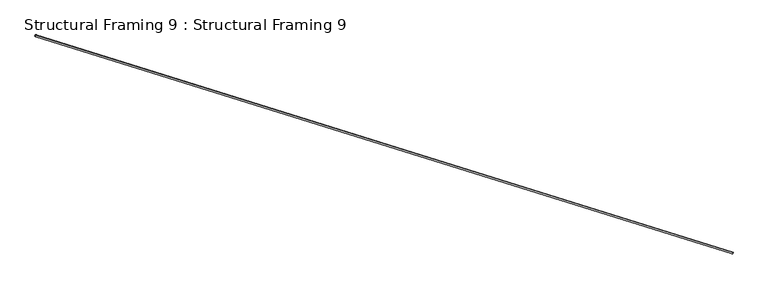
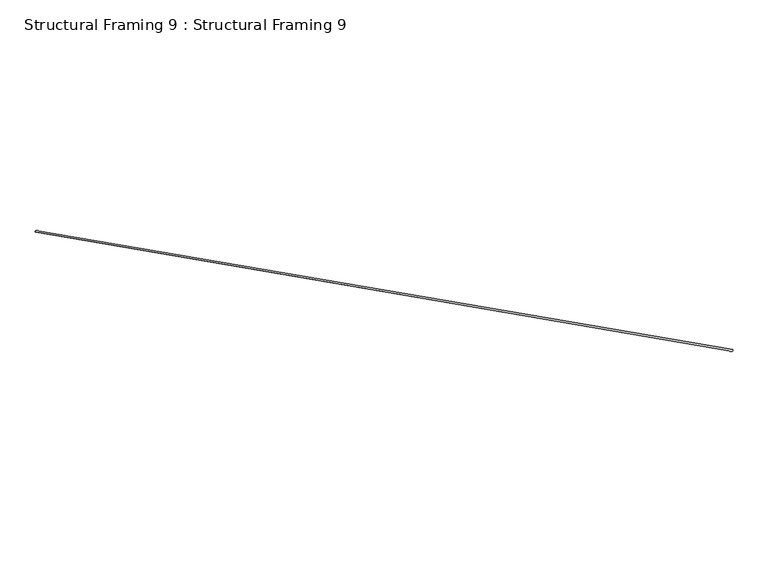
"""IFC4 building model written with IfcOpenShell, lengths in millimetres: beam geometry, Structural Framing 9 : Structural Framing 9."""

from ifc_helpers import new_model, si_unit, point, frame, origin, origin_2d, place, context, project, spatial, circle_curve, trimmed, segment, composite_curve, outline, extrude, source, transform, mapped, element, save


def structural_framing_9_structural_framing_9_9f5ad4d8(model_context):
    return source(origin(), model_context, "Body", "SweptSolid", [
        extrude(outline(composite_curve([segment(trimmed(circle_curve(origin_2d(), 6.35), [point((0.0, 6.35))], [point((0.0, -6.35))], False, "CARTESIAN"), True, "CONTINUOUS"), segment(trimmed(circle_curve(origin_2d(), 6.35), [point((0.0, -6.35))], [point((0.0, 6.35))], False, "CARTESIAN"), True, "CONTINUOUS")], self_intersect=False)), frame((17936.6160052, 2538.5077975, 2956.2008394), z_axis=(-0.8989286779363532, 0.2804615867326995, 0.33655390407923735), x_axis=(0.0, 0.7682212795973775, -0.6401843996644779)), (0.0, 0.0, 1.0), 5845.7129347),
    ])


if __name__ == "__main__":
    model = new_model("IFC4")
    model_context = context("Model", 3, world=origin())
    ifc_project = project(units=[si_unit("LENGTHUNIT", "METRE", prefix="MILLI")], contexts=[model_context])
    site = spatial("IfcSite", under=ifc_project)
    building = spatial("IfcBuilding", under=site)
    placement = place(None, origin())
    structural_framing_9_structural_framing_9_shape = structural_framing_9_structural_framing_9_9f5ad4d8(model_context)
    element("IfcBeam", 1, ObjectType="Structural Framing 9 : Structural Framing 9", at=placement, inside=building, context=model_context, shape_type="MappedRepresentation", body=[
        mapped(structural_framing_9_structural_framing_9_shape, transform((0.0, 0.0, 0.0), x_axis=(1.0, 0.0, 0.0), y_axis=(0.0, 1.0, 0.0), z_axis=(0.0, 0.0, 1.0))),
    ])
    save(model, "model.ifc")

# Revit data of these elements
# Type "Structural Framing 9 : Structural Framing 9"
#   Structural Material [instance default] = EXISTING LATERAL BRACING (1/4" CABLE)
# Element 1 (IfcBeam, "Structural Framing 9 : Structural Framing 9")
#   Materials on its faces: "EXISTING LATERAL BRACING (1/4\" CABLE)"
# Materials
#   "EXISTING LATERAL BRACING (1/4\" CABLE)": class "Generic", colour RGB 120 120 120, transparency 0, Cost = 0
